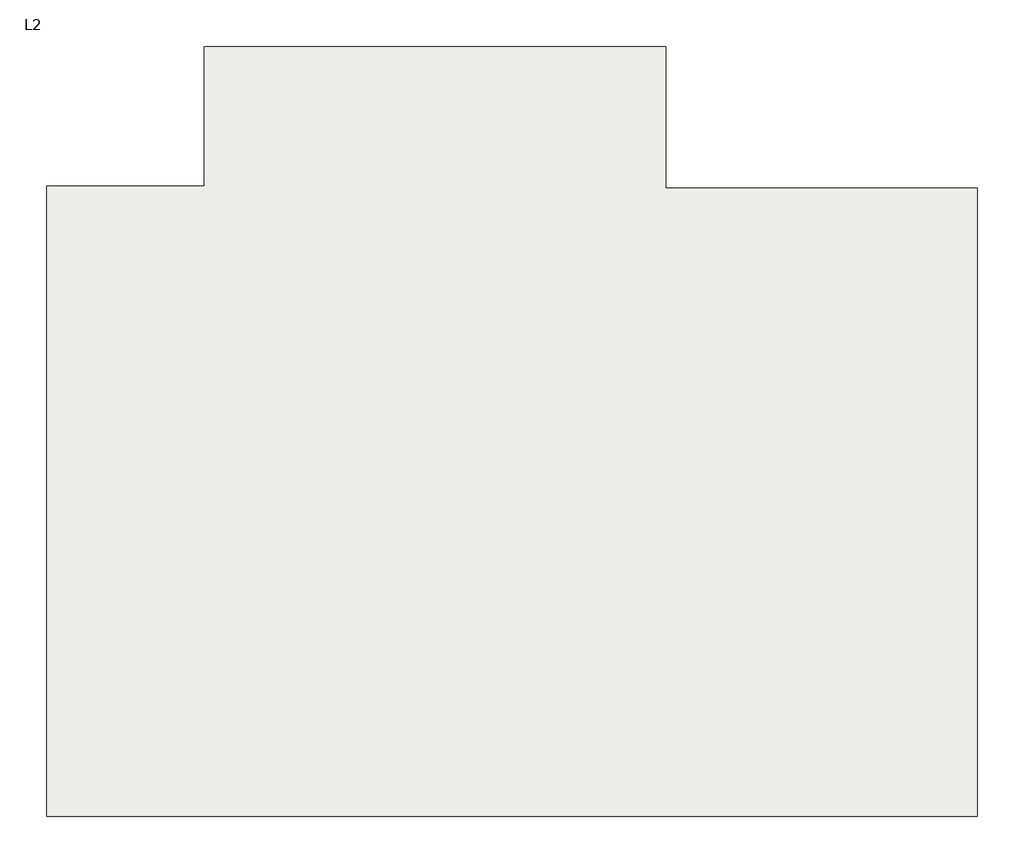
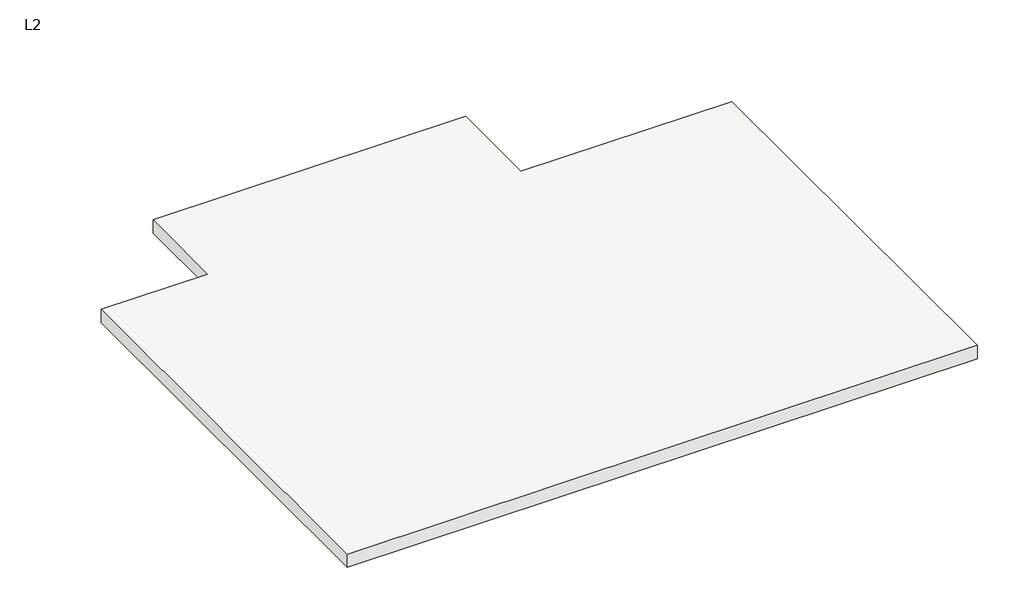
# One storey: 6 coverings, 1 roof.
"""IFC4 building model written with IfcOpenShell, lengths in millimetres."""

import ifcopenshell
import ifcopenshell.guid

model = None  # the IFC model being written
_history = None  # IfcOwnerHistory: only IFC2X3 demands one
_inside = {}  # id of a spatial element -> (the spatial element, [elements in it])
_under = {}  # id of a project, library or spatial element -> (it, [spatial elements below it])
_declared = {}  # id of a project -> (the project, [libraries it declares])
_typed = {}  # id of a type object -> (the type object, [elements of that type])
_made_of = {}  # id of a material, layer set ... -> (it, [elements and type objects made of it])


def new_model(schema):
    """Start an empty IFC model of exactly this schema.

    Asked for "IFC4X3", IfcOpenShell would pick the latest addendum, in which some entities
    have other attributes; the version numbers below select the first issue.
    IFC2X3 requires an IfcOwnerHistory on every rooted entity: one is made here for all.
    """
    global model, _history
    if schema == "IFC4X3":
        model = ifcopenshell.file(schema_version=(4, 3, 0, 0))
    else:
        model = ifcopenshell.file(schema=schema)
    _inside.clear()
    _under.clear()
    _declared.clear()
    _typed.clear()
    _made_of.clear()
    _history = None
    if model.schema == "IFC2X3":
        org = make("IfcOrganization", Name="unknown")
        user = make(
            "IfcPersonAndOrganization",
            ThePerson=make("IfcPerson", FamilyName="unknown"),
            TheOrganization=org,
        )
        app = make(
            "IfcApplication",
            ApplicationDeveloper=org,
            Version="unknown",
            ApplicationFullName="unknown",
            ApplicationIdentifier="unknown",
        )
        _history = make(
            "IfcOwnerHistory",
            OwningUser=user,
            OwningApplication=app,
            ChangeAction="ADDED",
            CreationDate=0,
        )
    return model


def make(cls, **values):
    """One entity of the class cls with the attributes given. An attribute that is None is left unset."""
    return model.create_entity(
        cls, **{name: value for name, value in values.items() if value is not None}
    )


def rooted(cls, **values):
    """An entity with a GlobalId (a new one), such as an element, a storey or a relation."""
    return make(cls, GlobalId=ifcopenshell.guid.new(), OwnerHistory=_history, **values)


def si_unit(unit_type, name, prefix=None):
    """IfcSIUnit, for example si_unit("LENGTHUNIT", "METRE", prefix="MILLI")."""
    return make("IfcSIUnit", UnitType=unit_type, Prefix=prefix, Name=name)


def assignment(units):
    """IfcUnitAssignment: the units of a project."""
    return None if units is None else make("IfcUnitAssignment", Units=units)


def point(xyz):
    """IfcCartesianPoint."""
    return None if xyz is None else make("IfcCartesianPoint", Coordinates=xyz)


def direction(xyz):
    """IfcDirection."""
    return None if xyz is None else make("IfcDirection", DirectionRatios=xyz)


def frame(location, z_axis=None, x_axis=None):
    """IfcAxis2Placement3D, a coordinate frame: its origin and axes. An axis left out is left unset."""
    return make(
        "IfcAxis2Placement3D",
        Location=point(location),
        Axis=direction(z_axis),
        RefDirection=direction(x_axis),
    )


def origin():
    """The frame at (0, 0, 0) with its axes left unset."""
    return frame((0.0, 0.0, 0.0))


def place(relative_to, where):
    """IfcLocalPlacement: puts the frame where relative to a parent placement (None: the world)."""
    return make(
        "IfcLocalPlacement", PlacementRelTo=relative_to, RelativePlacement=where
    )


def context(
    kind, dimensions, precision=None, world=None, true_north=None, identifier=None
):
    """IfcGeometricRepresentationContext, for example the 3D "Model" context."""
    return make(
        "IfcGeometricRepresentationContext",
        ContextIdentifier=identifier,
        ContextType=kind,
        CoordinateSpaceDimension=dimensions,
        Precision=precision,
        WorldCoordinateSystem=world,
        TrueNorth=true_north,
    )


def project(units=None, contexts=None):
    """IfcProject with its units and contexts."""
    return rooted(
        "IfcProject",
        Name="project",
        RepresentationContexts=contexts,
        UnitsInContext=assignment(units),
    )


def spatial(cls, under=None, at=None, **own):
    """A site, building, storey or space (cls), placed at a placement, below another one or the project."""
    s = rooted(cls, ObjectPlacement=at, **own)
    if under is not None:
        _under.setdefault(under.id(), (under, []))[1].append(s)
    return s


def polyline(points):
    """IfcPolyline through the points."""
    return make("IfcPolyline", Points=[point(p) for p in points])


def outline(outer, holes=None, kind="AREA"):
    """IfcArbitraryClosedProfileDef: a profile drawn as a closed curve; with holes, ...WithVoids."""
    if holes is None:
        return make("IfcArbitraryClosedProfileDef", ProfileType=kind, OuterCurve=outer)
    return make(
        "IfcArbitraryProfileDefWithVoids",
        ProfileType=kind,
        OuterCurve=outer,
        InnerCurves=holes,
    )


def extrude(swept, where, along, depth):
    """IfcExtrudedAreaSolid: the profile swept, set in the frame where, extruded along a direction by depth."""
    return make(
        "IfcExtrudedAreaSolid",
        SweptArea=swept,
        Position=where,
        ExtrudedDirection=direction(along),
        Depth=depth,
    )


def shape(context_of_items, identifier, shape_type, items):
    """IfcShapeRepresentation: the items that make up one representation, for example the "Body"."""
    return make(
        "IfcShapeRepresentation",
        ContextOfItems=context_of_items,
        RepresentationIdentifier=identifier,
        RepresentationType=shape_type,
        Items=items,
    )


def made_of(thing, what):
    """Note that an element or type object is made of a material, layer set ...; save() writes the relation."""
    if what is not None:
        _made_of.setdefault(what.id(), (what, []))[1].append(thing)
    return thing


def element(
    cls,
    number,
    at=None,
    inside=None,
    cuts=None,
    type_object=None,
    material=None,
    context=None,
    identifier="Body",
    shape_type=None,
    held_by="IfcProductDefinitionShape",
    body=None,
    shapes=None,
    **own,
):
    """One element of the class cls, such as IfcWall. Its Tag is "e" and its number.

    at: its placement. inside: the storey or other place that contains it. cuts: it is an
    opening in that element (IfcRelVoidsElement). A single representation is given by context,
    identifier, shape_type and body (its items); several are given by shapes. held_by: the class
    of the entity that holds the representations. save() writes the other relations.
    """
    e = rooted(cls, Tag="e%d" % number, ObjectPlacement=at, **own)
    if body is not None:
        shapes = [shape(context, identifier, shape_type, body)]
    if shapes is not None:
        e.Representation = make(held_by, Representations=shapes)
    if inside is not None:
        _inside.setdefault(inside.id(), (inside, []))[1].append(e)
    if cuts is not None:
        rooted(
            "IfcRelVoidsElement", RelatingBuildingElement=cuts, RelatedOpeningElement=e
        )
    if type_object is not None:
        _typed.setdefault(type_object.id(), (type_object, []))[1].append(e)
    return made_of(e, material)


def aggregate(whole, parts):
    """IfcRelAggregates: a whole, such as a stair, and the parts it consists of."""
    return rooted("IfcRelAggregates", RelatingObject=whole, RelatedObjects=parts)


def save(model, path):
    """Write the relations noted so far, then the file.

    IfcRelAggregates (storeys below a building ...), IfcRelContainedInSpatialStructure (elements
    in a storey), IfcRelDefinesByType, IfcRelAssociatesMaterial and IfcRelDeclares: one each for
    every whole, place, type object, material and project.
    """
    for whole, parts in _under.values():
        aggregate(whole, parts)
    for where, things in _inside.values():
        rooted(
            "IfcRelContainedInSpatialStructure",
            RelatedElements=things,
            RelatingStructure=where,
        )
    for kind, things in _typed.values():
        rooted("IfcRelDefinesByType", RelatedObjects=things, RelatingType=kind)
    for what, things in _made_of.values():
        rooted("IfcRelAssociatesMaterial", RelatedObjects=things, RelatingMaterial=what)
    for by, libraries in _declared.values():
        rooted("IfcRelDeclares", RelatingContext=by, RelatedDefinitions=libraries)
    model.write(path)


model = new_model("IFC4")

# Units and contexts
model_context = context("Model", 3, world=origin())
ifc_project = project(units=[si_unit("LENGTHUNIT", "METRE", prefix="MILLI")], contexts=[model_context])

# Site, building, storey
site = spatial("IfcSite", under=ifc_project)
building = spatial("IfcBuilding", under=site)
storey = spatial("IfcBuildingStorey", under=building, Name="L2", Elevation=4000.0)

# Coverings
placement = place(None, origin())
element("IfcCovering", 1, ObjectType="600mm x 600mm ACT System", at=placement, inside=storey, context=model_context, shape_type="SweptSolid", body=[
    extrude(outline(polyline([(-11010.0290877, -200.2324985), (-11010.0290877, 5740.7675015), (-7176.5290877, 5740.7675015), (-7176.5290877, -200.2324985), (-11010.0290877, -200.2324985)])), frame((0.0, 0.0, 3600.0), z_axis=(0.0, 0.0, 1.0), x_axis=(1.0, 0.0, 0.0)), (0.0, 0.0, 1.0), 56.0),
])
element("IfcCovering", 2, ObjectType="600mm x 600mm ACT System", at=placement, inside=storey, context=model_context, shape_type="SweptSolid", body=[
    extrude(outline(polyline([(-7051.5290877, -374.7324985), (-7051.5290877, 5915.2675015), (-6897.0290877, 5915.2675015), (-6897.0290877, 9391.7675015), (3950.9709123, 9391.7675015), (3950.9709123, 5866.2675015), (4033.4709123, 5866.2675015), (4033.4709123, -466.7324985), (-6910.0290877, -466.7324985), (-6910.0290877, -374.7324985), (-7051.5290877, -374.7324985)])), frame((0.0, 0.0, 3600.0), z_axis=(0.0, 0.0, 1.0), x_axis=(1.0, 0.0, 0.0)), (0.0, 0.0, 1.0), 56.0),
])
element("IfcCovering", 3, ObjectType="600mm x 600mm ACT System", at=placement, inside=storey, context=model_context, shape_type="SweptSolid", body=[
    extrude(outline(polyline([(4158.4709123, 5691.7675015), (12091.9709123, 5691.7675015), (12091.9709123, 1918.2675015), (4158.4709123, 1918.2675015), (4158.4709123, 5691.7675015)])), frame((0.0, 0.0, 3600.0), z_axis=(0.0, 0.0, 1.0), x_axis=(1.0, 0.0, 0.0)), (0.0, 0.0, 1.0), 56.0),
])
element("IfcCovering", 4, ObjectType="600mm x 600mm ACT System", at=placement, inside=storey, context=model_context, shape_type="SweptSolid", body=[
    extrude(outline(polyline([(4158.4709123, 1793.2675015), (12091.9709123, 1793.2675015), (12091.9709123, -5506.7324985), (4158.4709123, -5506.7324985), (4158.4709123, 1793.2675015)])), frame((0.0, 0.0, 3600.0), z_axis=(0.0, 0.0, 1.0), x_axis=(1.0, 0.0, 0.0)), (0.0, 0.0, 1.0), 56.0),
])
element("IfcCovering", 5, ObjectType="600mm x 600mm ACT System", at=placement, inside=storey, context=model_context, shape_type="SweptSolid", body=[
    extrude(outline(polyline([(12091.9709123, -5631.7324985), (12091.9709123, -9510.2324985), (4158.4709123, -9510.2324985), (4158.4709123, -5631.7324985), (12091.9709123, -5631.7324985)])), frame((0.0, 0.0, 3600.0), z_axis=(0.0, 0.0, 1.0), x_axis=(1.0, 0.0, 0.0)), (0.0, 0.0, 1.0), 56.0),
])
element("IfcCovering", 6, ObjectType="600mm x 600mm ACT System", at=placement, inside=storey, context=model_context, shape_type="SweptSolid", body=[
    extrude(outline(polyline([(-310.0290877, -6210.2324985), (-6910.0290877, -6210.2324985), (-6910.0290877, -591.7324985), (4033.4709123, -591.7324985), (4033.4709123, -9510.2324985), (-310.0290877, -9510.2324985), (-310.0290877, -6210.2324985)])), frame((0.0, 0.0, 3600.0), z_axis=(0.0, 0.0, 1.0), x_axis=(1.0, 0.0, 0.0)), (0.0, 0.0, 1.0), 56.0),
])

# Roof
element("IfcRoof", 7, ObjectType="M_Steel Truss - Insulation on Metal Deck - EPDM", at=placement, inside=storey, context=model_context, shape_type="SweptSolid", body=[
    extrude(outline(polyline([(12690.9709123, -10109.2324985), (-11609.0290877, -10109.2324985), (-11609.0290877, 6339.7675015), (-7496.5290877, 6339.7675015), (-7496.5290877, 9990.7675015), (4549.9709123, 9990.7675015), (4549.9709123, 6290.7675015), (12690.9709123, 6290.7675015), (12690.9709123, -10109.2324985)])), frame((0.0, 0.0, 4000.0), z_axis=(0.0, 0.0, 1.0), x_axis=(1.0, 0.0, 0.0)), (0.0, 0.0, 1.0), 537.0),
])

save(model, "model.ifc")

# Revit data of these elements
# Project information
#   Organization Name = "Organization Name"
#   Organization Description = "Organization Description"
#   Building Name = "Building Name"
#   Project Issue Date = "Issue Date"
#   Project Status = "Project Status"
#   Client Name = "Client Name"
#   Project Address = "Enter address here\nAddress Line 2"
#   Project Name = "Project Name"
#   Project Number = "Project Number"
# Type "600mm x 600mm ACT System"
#   Description = "24\" x 24\" Acoustical Ceiling Tile (ACT)"
#   Assembly Code = "C3030210"
#   Type Mark = "C03"
#   built-in parameter 1002203 = 1 (stored number, unit not read)
#   built-in parameter 1002202 = 1 (stored number, unit not read)
#   Layers, outside or top first: 40 mm "Default" (function 1); 16 mm "Acoustic Ceiling Tile 600 x 600" (function 5)
# Type "M_Steel Truss - Insulation on Metal Deck - EPDM"
#   Description = "Steel Deck with Metal Deck and Insultation and Ethylene Propylene Diene Monomer (EPDM) Finish"
#   Assembly Code = "B1020"
#   Type Mark = "R06"
#   Layers, outside or top first: 6 mm "Roofing, EPDM Membrane" (function 4); 125 mm "Rigid insulation" (function 3); 6 mm "Metal Deck" (function 1); 400 mm "Structure, Steel Bar Joist Layer" (function 1)
# Elements 1, 2, 3, 4, 5, 6 (IfcCovering, "600mm x 600mm ACT System")
#   Height Offset From Level = -400 mm
#   Phase Created = New Construction
#   Materials on its faces: "Acoustic Ceiling Tile 600 x 600", "Default"
# Element 7 (IfcRoof, "M_Steel Truss - Insulation on Metal Deck - EPDM")
#   built-in parameter 1001705 = 14.8852 (stored number, unit not read)
#   built-in parameter 1001710 = 33615
#   Phase Created = New Construction
#   Materials on its faces: "Structure, Steel Bar Joist Layer", "Roofing, EPDM Membrane"
# Materials
#   "Default": class "Miscellaneous", colour RGB 192 192 192, transparency 0, Cost = 0
#   "Acoustic Ceiling Tile 600 x 600": class "Generic", colour RGB 218 218 218, transparency 0, Description = "Acoustic Ceiling Tile 24 x 24", Cost = 0
#   "Roofing, EPDM Membrane": class "Generic", colour RGB 37 37 37, transparency 0, Description = "EPDM roof membrane", Cost = 0
#   "Rigid insulation": class "Generic", colour RGB 231 231 231, transparency 0, Description = "Rigid foam insulation board", Cost = 0
#   "Metal Deck": class "Metal", colour RGB 144 145 139, transparency 0, Description = "Steel, mill finish", Cost = 0
#   "Structure, Steel Bar Joist Layer": class "Metal", colour RGB 159 159 159, transparency 0, Description = "Bar joists, thermal airspace", Cost = 0
